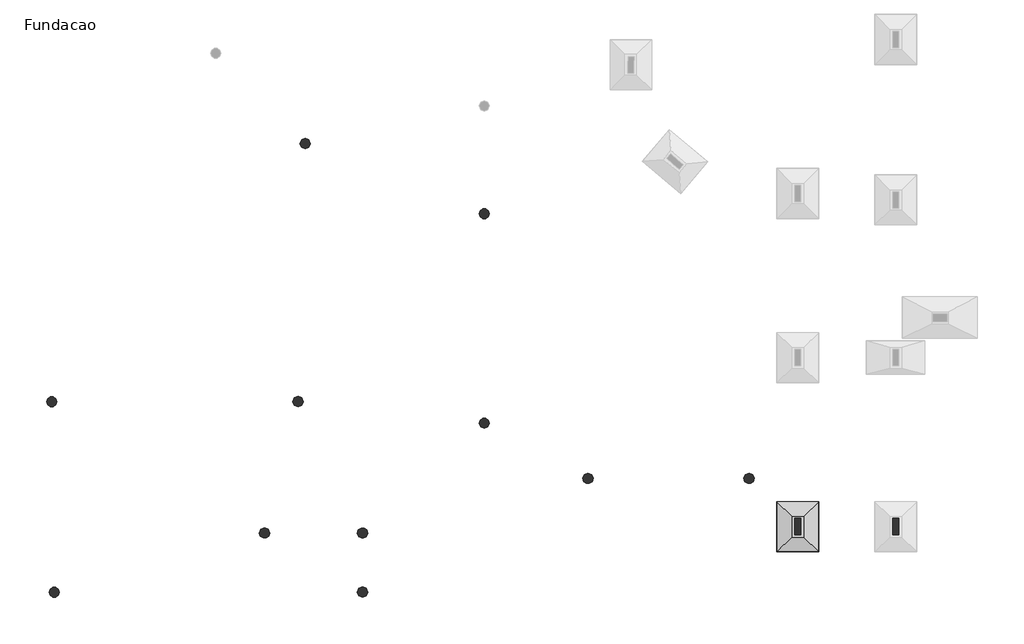
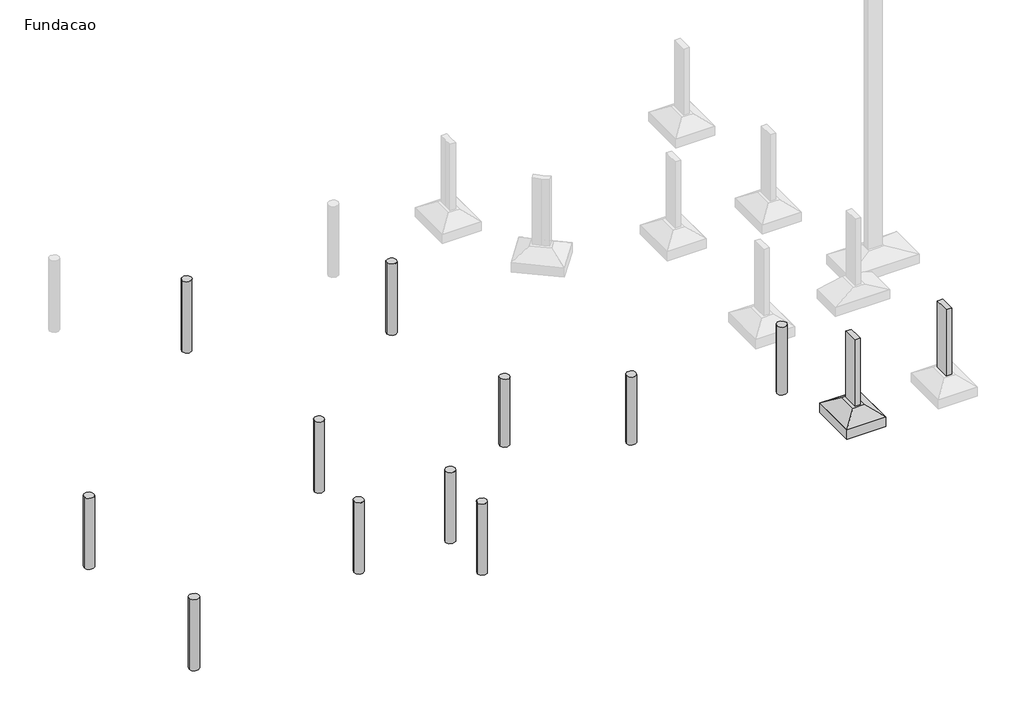
# One storey, part 1 of 2: 13 columns, 1 fastener.
# Revit data of these elements (continued)
# Element 12 (IfcColumn, "TQS - Pilar retangular : 14.0 x 40.0") (continued)
#   Pino = ""
#   Distribuicao = ""
#   Solidarizado = ""
#   Solidarizar na montagem = ""
#   Unir com o próximo = ""
#   Grupo pre moldado = ""
#   Verificado = ""
#   Concreto C = ""
#   Taxa de armadura (kgf/m³) = 0
#   Carga (tf/m²) = 0
#   Carga (tf/m) = 0
#   Carga (tf) = 0
#   Altura = 1.70 m
#   Rebaixo = 0.00 m
#   Altura da fundacao = 0.00 m
#   Largura = 0.00 m
#   Distancia a face = 0.00 m
#   Distancia ao eixo = 0.00 m
#   Resultado de Ensaios fck (MPa) = 0
#   Unique TQS ID = -966
#   Principal = yes
#   Nasce = yes
#   Morre = yes
#   Cabeca de Pilar = no
#   Structural Material = Concrete - Cast-in-Place Concrete
#   Phase Created = CC_AP/ESTR
#   Materials on its faces: "Concrete - Cast-in-Place Concrete"
# Element 13 (IfcColumn, "TQS - Pilar retangular : 14.0 x 40.0")
#   Uso = "ESTRUTURA"
#   Titulo = "PS10"
#   Chave = "PS10//0"
#   Tipo Elemento = "Pilar"
#   SHA1 = "348E9EB98025B598649ED725E9A09005B776015E"
#   Revisão = ""
#   Tipo de carga = ""
#   Divisor de flexao = ""
#   Secao = "R 14/40 180°"
#   Configuracao = ""
#   Angulo (graus) = ""
#   Detalhamento = ""
#   Casos de vento manual = ""
#   Tipo = ""
#   Alcas = ""
#   Furos = ""
#   Pino = ""
#   Distribuicao = ""
#   Solidarizado = ""
#   Solidarizar na montagem = ""
#   Unir com o próximo = ""
#   Grupo pre moldado = ""
#   Verificado = ""
#   Concreto C = ""
#   Taxa de armadura (kgf/m³) = 0
#   Carga (tf/m²) = 0
#   Carga (tf/m) = 0
#   Carga (tf) = 0
#   Altura = 1.70 m
#   Rebaixo = 0.00 m
#   Altura da fundacao = 0.00 m
#   Largura = 0.00 m
#   Distancia a face = 0.00 m
#   Distancia ao eixo = 0.00 m
#   Resultado de Ensaios fck (MPa) = 0
#   Unique TQS ID = -967
#   Principal = yes
#   Nasce = yes
#   Morre = yes
#   Cabeca de Pilar = no
#   Structural Material = Concrete - Cast-in-Place Concrete
#   Phase Created = CC_AP/ESTR
#   Materials on its faces: "Concrete - Cast-in-Place Concrete"
# Element 14 (IfcFastener, "TQS - Sapata : SPS9")
#   Uso = "ESTRUTURA"
#   Titulo = "SPS9"
#   Chave = "-1542"
#   Tipo Elemento = "Fundação"
#   SHA1 = "96B98524968DB2A66F18ED7D1088E2BB9B4616C7"
#   Revisão = ""
#   Tipo de carga = ""
#   Divisor de flexao = ""
#   Secao = ""
#   Configuracao = ""
#   Angulo (graus) = ""
#   Detalhamento = ""
#   Casos de vento manual = ""
#   Tipo = "Sapata"
#   Dimensoes = "100.0,120.0"
#   Estacas = ""
#   Calice = ""
#   Rugosidade = ""
#   Alcas = ""
#   Furos = ""
#   Pino = ""
#   Distribuicao = ""
#   Solidarizado = ""
#   Solidarizar na montagem = ""
#   Unir com o próximo = ""
#   Grupo pre moldado = ""
#   Verificado = ""
#   Concreto C = ""
#   Taxa de armadura (kgf/m³) = 0
#   Carga (tf/m²) = 0
#   Carga (tf/m) = 0
#   Carga (tf) = 0
#   Altura = 0.00 m
#   Rebaixo = 0.00 m
#   Pilar ficticio = 0.00 m
#   Topo = -1.45 m
#   Altura total = 0.50 m
#   Rodape = 0.00 m
#   Diametro = 0.00 m
#   Altura dentro do bloco = 0.00 m
#   Entre eixos = 0.00 m
#   Paredes = 0.00 m
#   Caimento = 0.00 m
#   Largura = 0.00 m
#   Distancia a face = 0.00 m
#   Distancia ao eixo = 0.00 m
#   Resultado de Ensaios fck (MPa) = 0
#   Unique TQS ID = -1542
#   Principal = yes
#   Phase Created = CC_AP/ESTR
#   Materials on its faces: "Concreto - Concreto concretado no local"
# Materials
#   "Concrete - Cast-in-Place Concrete": class "Unassigned", colour RGB 192 192 192, transparency 0
#   "Concreto - Concreto concretado no local": class "Concreto", colour RGB 192 192 192, transparency 0
